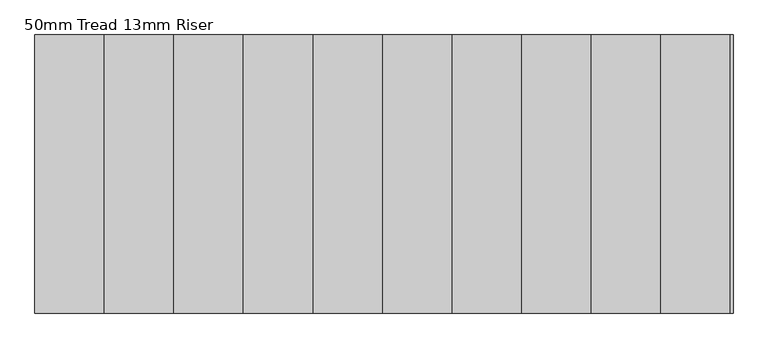
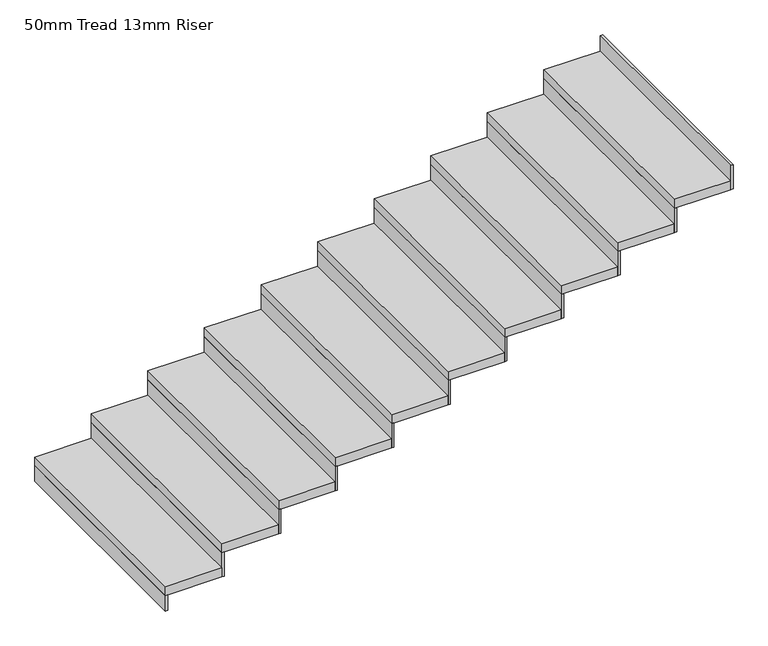
"""IFC4 building model written with IfcOpenShell, lengths in millimetres: stair flight geometry, 50mm Tread 13mm Riser."""

from ifc_helpers import new_model, si_unit, frame, origin, origin_with_axes, place, context, project, spatial, polyline, outline, extrude, source, transform, mapped, element, save


def stair_flight_50mm_tread_13mm_riser_5af3cbe2(model_context):
    return source(origin(), model_context, "Body", "SweptSolid", [
        extrude(outline(polyline([(-14715.2499729, -6081.4588442), (-14727.7499729, -6081.4588442), (-14727.7499729, -4881.4588442), (-14715.2499729, -4881.4588442), (-14715.2499729, -6081.4588442)])), origin_with_axes(), (0.0, 0.0, 1.0), 86.3636364),
        extrude(outline(polyline([(-14427.7499729, -4881.4588442), (-14427.7499729, -6081.4588442), (-14727.7499729, -6081.4588442), (-14727.7499729, -4881.4588442), (-14427.7499729, -4881.4588442)])), frame((0.0, 0.0, 86.3636364), z_axis=(0.0, 0.0, 1.0), x_axis=(1.0, 0.0, 0.0)), (0.0, 0.0, 1.0), 50.0),
        extrude(outline(polyline([(-14415.2499729, -6081.4588442), (-14427.7499729, -6081.4588442), (-14427.7499729, -4881.4588442), (-14415.2499729, -4881.4588442), (-14415.2499729, -6081.4588442)])), frame((0.0, 0.0, 86.3636364), z_axis=(0.0, 0.0, 1.0), x_axis=(1.0, 0.0, 0.0)), (0.0, 0.0, 1.0), 136.3636364),
        extrude(outline(polyline([(-14127.7499729, -4881.4588442), (-14127.7499729, -6081.4588442), (-14427.7499729, -6081.4588442), (-14427.7499729, -4881.4588442), (-14127.7499729, -4881.4588442)])), frame((0.0, 0.0, 222.7272727), z_axis=(0.0, 0.0, 1.0), x_axis=(1.0, 0.0, 0.0)), (0.0, 0.0, 1.0), 50.0),
        extrude(outline(polyline([(-14115.2499729, -6081.4588442), (-14127.7499729, -6081.4588442), (-14127.7499729, -4881.4588442), (-14115.2499729, -4881.4588442), (-14115.2499729, -6081.4588442)])), frame((0.0, 0.0, 222.7272727), z_axis=(0.0, 0.0, 1.0), x_axis=(1.0, 0.0, 0.0)), (0.0, 0.0, 1.0), 136.3636364),
        extrude(outline(polyline([(-13827.7499729, -4881.4588442), (-13827.7499729, -6081.4588442), (-14127.7499729, -6081.4588442), (-14127.7499729, -4881.4588442), (-13827.7499729, -4881.4588442)])), frame((0.0, 0.0, 359.0909091), z_axis=(0.0, 0.0, 1.0), x_axis=(1.0, 0.0, 0.0)), (0.0, 0.0, 1.0), 50.0),
        extrude(outline(polyline([(-13815.2499729, -6081.4588442), (-13827.7499729, -6081.4588442), (-13827.7499729, -4881.4588442), (-13815.2499729, -4881.4588442), (-13815.2499729, -6081.4588442)])), frame((0.0, 0.0, 359.0909091), z_axis=(0.0, 0.0, 1.0), x_axis=(1.0, 0.0, 0.0)), (0.0, 0.0, 1.0), 136.3636364),
        extrude(outline(polyline([(-13527.7499729, -4881.4588442), (-13527.7499729, -6081.4588442), (-13827.7499729, -6081.4588442), (-13827.7499729, -4881.4588442), (-13527.7499729, -4881.4588442)])), frame((0.0, 0.0, 495.4545455), z_axis=(0.0, 0.0, 1.0), x_axis=(1.0, 0.0, 0.0)), (0.0, 0.0, 1.0), 50.0),
        extrude(outline(polyline([(-13515.2499729, -6081.4588442), (-13527.7499729, -6081.4588442), (-13527.7499729, -4881.4588442), (-13515.2499729, -4881.4588442), (-13515.2499729, -6081.4588442)])), frame((0.0, 0.0, 495.4545455), z_axis=(0.0, 0.0, 1.0), x_axis=(1.0, 0.0, 0.0)), (0.0, 0.0, 1.0), 136.3636364),
        extrude(outline(polyline([(-13227.7499729, -4881.4588442), (-13227.7499729, -6081.4588442), (-13527.7499729, -6081.4588442), (-13527.7499729, -4881.4588442), (-13227.7499729, -4881.4588442)])), frame((0.0, 0.0, 631.8181818), z_axis=(0.0, 0.0, 1.0), x_axis=(1.0, 0.0, 0.0)), (0.0, 0.0, 1.0), 50.0),
        extrude(outline(polyline([(-13215.2499729, -6081.4588442), (-13227.7499729, -6081.4588442), (-13227.7499729, -4881.4588442), (-13215.2499729, -4881.4588442), (-13215.2499729, -6081.4588442)])), frame((0.0, 0.0, 631.8181818), z_axis=(0.0, 0.0, 1.0), x_axis=(1.0, 0.0, 0.0)), (0.0, 0.0, 1.0), 136.3636364),
        extrude(outline(polyline([(-12927.7499729, -4881.4588442), (-12927.7499729, -6081.4588442), (-13227.7499729, -6081.4588442), (-13227.7499729, -4881.4588442), (-12927.7499729, -4881.4588442)])), frame((0.0, 0.0, 768.1818182), z_axis=(0.0, 0.0, 1.0), x_axis=(1.0, 0.0, 0.0)), (0.0, 0.0, 1.0), 50.0),
        extrude(outline(polyline([(-12915.2499729, -6081.4588442), (-12927.7499729, -6081.4588442), (-12927.7499729, -4881.4588442), (-12915.2499729, -4881.4588442), (-12915.2499729, -6081.4588442)])), frame((0.0, 0.0, 768.1818182), z_axis=(0.0, 0.0, 1.0), x_axis=(1.0, 0.0, 0.0)), (0.0, 0.0, 1.0), 136.3636364),
        extrude(outline(polyline([(-12627.7499729, -4881.4588442), (-12627.7499729, -6081.4588442), (-12927.7499729, -6081.4588442), (-12927.7499729, -4881.4588442), (-12627.7499729, -4881.4588442)])), frame((0.0, 0.0, 904.5454545), z_axis=(0.0, 0.0, 1.0), x_axis=(1.0, 0.0, 0.0)), (0.0, 0.0, 1.0), 50.0),
        extrude(outline(polyline([(-12615.2499729, -6081.4588442), (-12627.7499729, -6081.4588442), (-12627.7499729, -4881.4588442), (-12615.2499729, -4881.4588442), (-12615.2499729, -6081.4588442)])), frame((0.0, 0.0, 904.5454545), z_axis=(0.0, 0.0, 1.0), x_axis=(1.0, 0.0, 0.0)), (0.0, 0.0, 1.0), 136.3636364),
        extrude(outline(polyline([(-12327.7499729, -4881.4588442), (-12327.7499729, -6081.4588442), (-12627.7499729, -6081.4588442), (-12627.7499729, -4881.4588442), (-12327.7499729, -4881.4588442)])), frame((0.0, 0.0, 1040.9090909), z_axis=(0.0, 0.0, 1.0), x_axis=(1.0, 0.0, 0.0)), (0.0, 0.0, 1.0), 50.0),
        extrude(outline(polyline([(-12315.2499729, -6081.4588442), (-12327.7499729, -6081.4588442), (-12327.7499729, -4881.4588442), (-12315.2499729, -4881.4588442), (-12315.2499729, -6081.4588442)])), frame((0.0, 0.0, 1040.9090909), z_axis=(0.0, 0.0, 1.0), x_axis=(1.0, 0.0, 0.0)), (0.0, 0.0, 1.0), 136.3636364),
        extrude(outline(polyline([(-12027.7499729, -4881.4588442), (-12027.7499729, -6081.4588442), (-12327.7499729, -6081.4588442), (-12327.7499729, -4881.4588442), (-12027.7499729, -4881.4588442)])), frame((0.0, 0.0, 1177.2727273), z_axis=(0.0, 0.0, 1.0), x_axis=(1.0, 0.0, 0.0)), (0.0, 0.0, 1.0), 50.0),
        extrude(outline(polyline([(-12015.2499729, -6081.4588442), (-12027.7499729, -6081.4588442), (-12027.7499729, -4881.4588442), (-12015.2499729, -4881.4588442), (-12015.2499729, -6081.4588442)])), frame((0.0, 0.0, 1177.2727273), z_axis=(0.0, 0.0, 1.0), x_axis=(1.0, 0.0, 0.0)), (0.0, 0.0, 1.0), 136.3636364),
        extrude(outline(polyline([(-11715.2499729, -6081.4588442), (-11727.7499729, -6081.4588442), (-11727.7499729, -4881.4588442), (-11715.2499729, -4881.4588442), (-11715.2499729, -6081.4588442)])), frame((0.0, 0.0, 1313.6363636), z_axis=(0.0, 0.0, 1.0), x_axis=(1.0, 0.0, 0.0)), (0.0, 0.0, 1.0), 136.3636364),
        extrude(outline(polyline([(-11727.7499729, -4881.4588442), (-11727.7499729, -6081.4588442), (-12027.7499729, -6081.4588442), (-12027.7499729, -4881.4588442), (-11727.7499729, -4881.4588442)])), frame((0.0, 0.0, 1313.6363636), z_axis=(0.0, 0.0, 1.0), x_axis=(1.0, 0.0, 0.0)), (0.0, 0.0, 1.0), 50.0),
    ])


if __name__ == "__main__":
    model = new_model("IFC4")
    model_context = context("Model", 3, world=origin())
    ifc_project = project(units=[si_unit("LENGTHUNIT", "METRE", prefix="MILLI")], contexts=[model_context])
    site = spatial("IfcSite", under=ifc_project)
    building = spatial("IfcBuilding", under=site)
    placement = place(None, origin())
    stair_flight_50mm_tread_13mm_riser_shape = stair_flight_50mm_tread_13mm_riser_5af3cbe2(model_context)
    element("IfcStairFlight", 1, ObjectType="50mm Tread 13mm Riser", at=placement, inside=building, context=model_context, shape_type="MappedRepresentation", body=[
        mapped(stair_flight_50mm_tread_13mm_riser_shape, transform((0.0, 0.0, 0.0), x_axis=(1.0, 0.0, 0.0), y_axis=(0.0, 1.0, 0.0), z_axis=(0.0, 0.0, 1.0))),
    ])
    save(model, "model.ifc")
